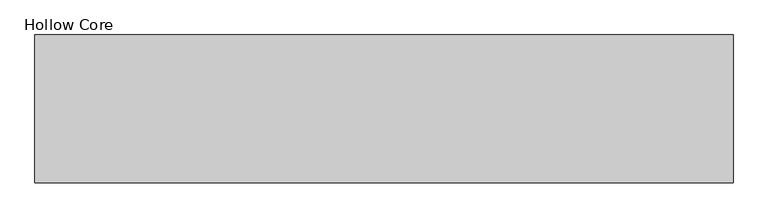
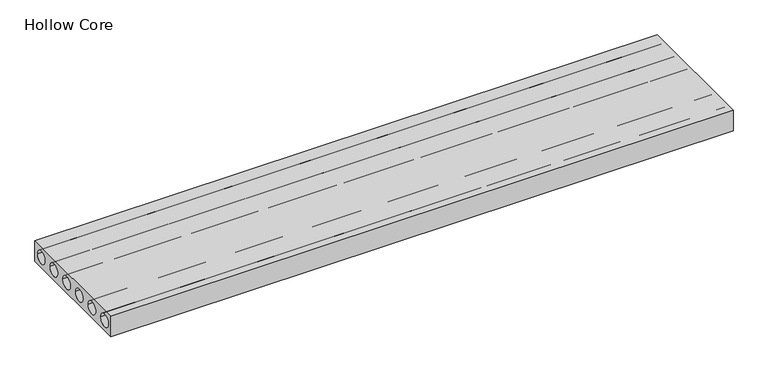
"""IFC4 building model written with IfcOpenShell, lengths in millimetres: proxy geometry, Hollow Core : Breton Hollow Core."""

import ifcopenshell
import ifcopenshell.guid

model = None  # the IFC model being written
_history = None  # IfcOwnerHistory: only IFC2X3 demands one
_inside = {}  # id of a spatial element -> (the spatial element, [elements in it])
_under = {}  # id of a project, library or spatial element -> (it, [spatial elements below it])
_declared = {}  # id of a project -> (the project, [libraries it declares])
_typed = {}  # id of a type object -> (the type object, [elements of that type])
_made_of = {}  # id of a material, layer set ... -> (it, [elements and type objects made of it])


def new_model(schema):
    """Start an empty IFC model of exactly this schema.

    Asked for "IFC4X3", IfcOpenShell would pick the latest addendum, in which some entities
    have other attributes; the version numbers below select the first issue.
    IFC2X3 requires an IfcOwnerHistory on every rooted entity: one is made here for all.
    """
    global model, _history
    if schema == "IFC4X3":
        model = ifcopenshell.file(schema_version=(4, 3, 0, 0))
    else:
        model = ifcopenshell.file(schema=schema)
    _inside.clear()
    _under.clear()
    _declared.clear()
    _typed.clear()
    _made_of.clear()
    _history = None
    if model.schema == "IFC2X3":
        org = make("IfcOrganization", Name="unknown")
        user = make(
            "IfcPersonAndOrganization",
            ThePerson=make("IfcPerson", FamilyName="unknown"),
            TheOrganization=org,
        )
        app = make(
            "IfcApplication",
            ApplicationDeveloper=org,
            Version="unknown",
            ApplicationFullName="unknown",
            ApplicationIdentifier="unknown",
        )
        _history = make(
            "IfcOwnerHistory",
            OwningUser=user,
            OwningApplication=app,
            ChangeAction="ADDED",
            CreationDate=0,
        )
    return model


def make(cls, **values):
    """One entity of the class cls with the attributes given. An attribute that is None is left unset."""
    return model.create_entity(
        cls, **{name: value for name, value in values.items() if value is not None}
    )


def rooted(cls, **values):
    """An entity with a GlobalId (a new one), such as an element, a storey or a relation."""
    return make(cls, GlobalId=ifcopenshell.guid.new(), OwnerHistory=_history, **values)


def si_unit(unit_type, name, prefix=None):
    """IfcSIUnit, for example si_unit("LENGTHUNIT", "METRE", prefix="MILLI")."""
    return make("IfcSIUnit", UnitType=unit_type, Prefix=prefix, Name=name)


def assignment(units):
    """IfcUnitAssignment: the units of a project."""
    return None if units is None else make("IfcUnitAssignment", Units=units)


def point(xyz):
    """IfcCartesianPoint."""
    return None if xyz is None else make("IfcCartesianPoint", Coordinates=xyz)


def direction(xyz):
    """IfcDirection."""
    return None if xyz is None else make("IfcDirection", DirectionRatios=xyz)


def frame(location, z_axis=None, x_axis=None):
    """IfcAxis2Placement3D, a coordinate frame: its origin and axes. An axis left out is left unset."""
    return make(
        "IfcAxis2Placement3D",
        Location=point(location),
        Axis=direction(z_axis),
        RefDirection=direction(x_axis),
    )


def frame_2d(location, x_axis=None):
    """IfcAxis2Placement2D, a coordinate frame in the plane: its origin and x axis."""
    return make(
        "IfcAxis2Placement2D", Location=point(location), RefDirection=direction(x_axis)
    )


def origin():
    """The frame at (0, 0, 0) with its axes left unset."""
    return frame((0.0, 0.0, 0.0))


def place(relative_to, where):
    """IfcLocalPlacement: puts the frame where relative to a parent placement (None: the world)."""
    return make(
        "IfcLocalPlacement", PlacementRelTo=relative_to, RelativePlacement=where
    )


def context(
    kind, dimensions, precision=None, world=None, true_north=None, identifier=None
):
    """IfcGeometricRepresentationContext, for example the 3D "Model" context."""
    return make(
        "IfcGeometricRepresentationContext",
        ContextIdentifier=identifier,
        ContextType=kind,
        CoordinateSpaceDimension=dimensions,
        Precision=precision,
        WorldCoordinateSystem=world,
        TrueNorth=true_north,
    )


def project(units=None, contexts=None):
    """IfcProject with its units and contexts."""
    return rooted(
        "IfcProject",
        Name="project",
        RepresentationContexts=contexts,
        UnitsInContext=assignment(units),
    )


def spatial(cls, under=None, at=None, **own):
    """A site, building, storey or space (cls), placed at a placement, below another one or the project."""
    s = rooted(cls, ObjectPlacement=at, **own)
    if under is not None:
        _under.setdefault(under.id(), (under, []))[1].append(s)
    return s


def polyline(points):
    """IfcPolyline through the points."""
    return make("IfcPolyline", Points=[point(p) for p in points])


def circle_curve(where, radius):
    """IfcCircle in the frame where."""
    return make("IfcCircle", Position=where, Radius=radius)


def trimmed(basis, trim1, trim2, sense, master):
    """IfcTrimmedCurve: the piece of a basis curve between two trims."""
    return make(
        "IfcTrimmedCurve",
        BasisCurve=basis,
        Trim1=trim1,
        Trim2=trim2,
        SenseAgreement=sense,
        MasterRepresentation=master,
    )


def segment(curve, same_sense, transition):
    """IfcCompositeCurveSegment."""
    return make(
        "IfcCompositeCurveSegment",
        Transition=transition,
        SameSense=same_sense,
        ParentCurve=curve,
    )


def composite_curve(segments, self_intersect=None):
    """IfcCompositeCurve: segments joined end to end."""
    return make("IfcCompositeCurve", Segments=segments, SelfIntersect=self_intersect)


def outline(outer, holes=None, kind="AREA"):
    """IfcArbitraryClosedProfileDef: a profile drawn as a closed curve; with holes, ...WithVoids."""
    if holes is None:
        return make("IfcArbitraryClosedProfileDef", ProfileType=kind, OuterCurve=outer)
    return make(
        "IfcArbitraryProfileDefWithVoids",
        ProfileType=kind,
        OuterCurve=outer,
        InnerCurves=holes,
    )


def extrude(swept, where, along, depth):
    """IfcExtrudedAreaSolid: the profile swept, set in the frame where, extruded along a direction by depth."""
    return make(
        "IfcExtrudedAreaSolid",
        SweptArea=swept,
        Position=where,
        ExtrudedDirection=direction(along),
        Depth=depth,
    )


def shape(context_of_items, identifier, shape_type, items):
    """IfcShapeRepresentation: the items that make up one representation, for example the "Body"."""
    return make(
        "IfcShapeRepresentation",
        ContextOfItems=context_of_items,
        RepresentationIdentifier=identifier,
        RepresentationType=shape_type,
        Items=items,
    )


def source(mapping_origin, context_of_items, identifier, shape_type, items):
    """IfcRepresentationMap: a shape defined once, which mapped items show again and again."""
    return make(
        "IfcRepresentationMap",
        MappingOrigin=mapping_origin,
        MappedRepresentation=shape(context_of_items, identifier, shape_type, items),
    )


def transform(
    local_origin,
    x_axis=None,
    y_axis=None,
    z_axis=None,
    scale=None,
    scale2=None,
    scale3=None,
    uniform=True,
):
    """IfcCartesianTransformationOperator3D, or its non-uniform kind. x_axis, y_axis, z_axis: its Axis1, 2, 3."""
    if uniform:
        return make(
            "IfcCartesianTransformationOperator3D",
            Axis1=direction(x_axis),
            Axis2=direction(y_axis),
            LocalOrigin=point(local_origin),
            Scale=scale,
            Axis3=direction(z_axis),
        )
    return make(
        "IfcCartesianTransformationOperator3DnonUniform",
        Axis1=direction(x_axis),
        Axis2=direction(y_axis),
        LocalOrigin=point(local_origin),
        Scale=scale,
        Axis3=direction(z_axis),
        Scale2=scale2,
        Scale3=scale3,
    )


def mapped(mapping_source, mapping_target):
    """IfcMappedItem: shows the shape of a source again, moved by a transform."""
    return make(
        "IfcMappedItem", MappingSource=mapping_source, MappingTarget=mapping_target
    )


def made_of(thing, what):
    """Note that an element or type object is made of a material, layer set ...; save() writes the relation."""
    if what is not None:
        _made_of.setdefault(what.id(), (what, []))[1].append(thing)
    return thing


def element(
    cls,
    number,
    at=None,
    inside=None,
    cuts=None,
    type_object=None,
    material=None,
    context=None,
    identifier="Body",
    shape_type=None,
    held_by="IfcProductDefinitionShape",
    body=None,
    shapes=None,
    **own,
):
    """One element of the class cls, such as IfcWall. Its Tag is "e" and its number.

    at: its placement. inside: the storey or other place that contains it. cuts: it is an
    opening in that element (IfcRelVoidsElement). A single representation is given by context,
    identifier, shape_type and body (its items); several are given by shapes. held_by: the class
    of the entity that holds the representations. save() writes the other relations.
    """
    e = rooted(cls, Tag="e%d" % number, ObjectPlacement=at, **own)
    if body is not None:
        shapes = [shape(context, identifier, shape_type, body)]
    if shapes is not None:
        e.Representation = make(held_by, Representations=shapes)
    if inside is not None:
        _inside.setdefault(inside.id(), (inside, []))[1].append(e)
    if cuts is not None:
        rooted(
            "IfcRelVoidsElement", RelatingBuildingElement=cuts, RelatedOpeningElement=e
        )
    if type_object is not None:
        _typed.setdefault(type_object.id(), (type_object, []))[1].append(e)
    return made_of(e, material)


def aggregate(whole, parts):
    """IfcRelAggregates: a whole, such as a stair, and the parts it consists of."""
    return rooted("IfcRelAggregates", RelatingObject=whole, RelatedObjects=parts)


def save(model, path):
    """Write the relations noted so far, then the file.

    IfcRelAggregates (storeys below a building ...), IfcRelContainedInSpatialStructure (elements
    in a storey), IfcRelDefinesByType, IfcRelAssociatesMaterial and IfcRelDeclares: one each for
    every whole, place, type object, material and project.
    """
    for whole, parts in _under.values():
        aggregate(whole, parts)
    for where, things in _inside.values():
        rooted(
            "IfcRelContainedInSpatialStructure",
            RelatedElements=things,
            RelatingStructure=where,
        )
    for kind, things in _typed.values():
        rooted("IfcRelDefinesByType", RelatedObjects=things, RelatingType=kind)
    for what, things in _made_of.values():
        rooted("IfcRelAssociatesMaterial", RelatedObjects=things, RelatingMaterial=what)
    for by, libraries in _declared.values():
        rooted("IfcRelDeclares", RelatingContext=by, RelatedDefinitions=libraries)
    model.write(path)


def hollow_core_b1c9e8cf(model_context):
    return source(origin(), model_context, "Body", "SweptSolid", [
        extrude(outline(polyline([(-609.6, 100.0), (609.6, 100.0), (609.6, -100.0), (-609.6, -100.0), (-609.6, 100.0)]), holes=[composite_curve([segment(trimmed(circle_curve(frame_2d((508.0, 0.0)), 60.0), [point((448.0, 0.0))], [point((568.0, 0.0))], True, "CARTESIAN"), True, "CONTINUOUS"), segment(trimmed(circle_curve(frame_2d((508.0, 0.0)), 60.0), [point((568.0, 0.0))], [point((448.0, 0.0))], True, "CARTESIAN"), True, "CONTINUOUS")], self_intersect=False), composite_curve([segment(trimmed(circle_curve(frame_2d((-508.0, 0.0)), 60.0), [point((-568.0, 0.0))], [point((-448.0, 0.0))], True, "CARTESIAN"), True, "CONTINUOUS"), segment(trimmed(circle_curve(frame_2d((-508.0, 0.0)), 60.0), [point((-448.0, 0.0))], [point((-568.0, 0.0))], True, "CARTESIAN"), True, "CONTINUOUS")], self_intersect=False), composite_curve([segment(trimmed(circle_curve(frame_2d((304.8, 0.0)), 60.0), [point((244.8, 0.0))], [point((364.8, 0.0))], True, "CARTESIAN"), True, "CONTINUOUS"), segment(trimmed(circle_curve(frame_2d((304.8, 0.0)), 60.0), [point((364.8, 0.0))], [point((244.8, 0.0))], True, "CARTESIAN"), True, "CONTINUOUS")], self_intersect=False), composite_curve([segment(trimmed(circle_curve(frame_2d((101.6, 0.0)), 60.0), [point((41.6, 0.0))], [point((161.6, 0.0))], True, "CARTESIAN"), True, "CONTINUOUS"), segment(trimmed(circle_curve(frame_2d((101.6, 0.0)), 60.0), [point((161.6, 0.0))], [point((41.6, 0.0))], True, "CARTESIAN"), True, "CONTINUOUS")], self_intersect=False), composite_curve([segment(trimmed(circle_curve(frame_2d((-101.6, 0.0)), 60.0), [point((-161.6, 0.0))], [point((-41.6, 0.0))], True, "CARTESIAN"), True, "CONTINUOUS"), segment(trimmed(circle_curve(frame_2d((-101.6, 0.0)), 60.0), [point((-41.6, 0.0))], [point((-161.6, 0.0))], True, "CARTESIAN"), True, "CONTINUOUS")], self_intersect=False), composite_curve([segment(trimmed(circle_curve(frame_2d((-304.8, 0.0)), 60.0), [point((-364.8, 0.0))], [point((-244.8, 0.0))], True, "CARTESIAN"), True, "CONTINUOUS"), segment(trimmed(circle_curve(frame_2d((-304.8, 0.0)), 60.0), [point((-244.8, 0.0))], [point((-364.8, 0.0))], True, "CARTESIAN"), True, "CONTINUOUS")], self_intersect=False)]), frame((0.0, 0.0, 0.0), z_axis=(1.0, 0.0, 0.0), x_axis=(0.0, 1.0, 0.0)), (0.0, 0.0, 1.0), 5760.0),
    ])


if __name__ == "__main__":
    model = new_model("IFC4")
    model_context = context("Model", 3, world=origin())
    ifc_project = project(units=[si_unit("LENGTHUNIT", "METRE", prefix="MILLI")], contexts=[model_context])
    site = spatial("IfcSite", under=ifc_project)
    building = spatial("IfcBuilding", under=site)
    placement = place(None, origin())
    hollow_core_shape = hollow_core_b1c9e8cf(model_context)
    element("IfcBuildingElementProxy", 1, Name="Hollow Core : Breton Hollow Core", ObjectType="Hollow Core : Breton Hollow Core", at=placement, inside=building, context=model_context, shape_type="MappedRepresentation", body=[
        mapped(hollow_core_shape, transform((0.0, 0.0, 0.0), x_axis=(1.0, 0.0, 0.0), y_axis=(0.0, 1.0, 0.0), z_axis=(0.0, 0.0, 1.0))),
    ])
    save(model, "model.ifc")

# Revit data of these elements
# Type "Hollow Core : Breton Hollow Core"
#   Width [instance default] = 1219.2 mm
#   built-in parameter 1001306 [instance default] = 4 (stored number, unit not read)
#   Depth [instance default] = 152.4 mm
#   Core Radius [instance default] = 50.8 mm
#   Core Offset [instance default] = 101.6 mm
#   Number Of Cores [instance default] = 2
#   Material [instance default] = Concrete - Precast Concrete - Normal Weight - 5 ksi
#   Default Elevation = 0
#   Assembly Code = ""
# Element 1 (IfcBuildingElementProxy, "Hollow Core : Breton Hollow Core")
#   built-in parameter 1001306 = 18.8976 (stored number, unit not read)
#   Depth = 200 mm
#   Core Radius = 60 mm
#   Number Of Cores = 6
#   Materials on its faces: "Concrete - Precast Concrete - Normal Weight - 5 ksi"
# Materials
#   "Concrete - Precast Concrete - Normal Weight - 5 ksi": class "Concrete", colour RGB 198 187 187, transparency 0
